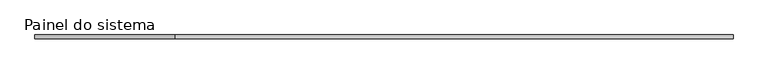
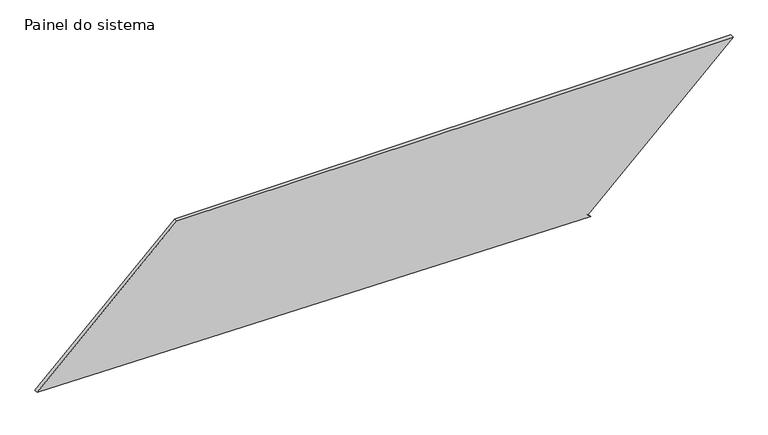
"""IFC4 building model written with IfcOpenShell, lengths in millimetres: plate geometry, Painel do sistema : Envidraçado."""

from ifc_helpers import new_model, si_unit, frame, origin, place, context, project, spatial, polyline, outline, extrude, source, transform, mapped, element, save


def painel_do_sistema_2f92d7f1(model_context):
    return source(origin(), model_context, "Body", "SweptSolid", [
        extrude(outline(polyline([(0.0, 1368.5356196), (18.146416, 1351.3394693), (933.8359883, 2317.6303845), (933.8359883, -1386.1476393), (51.1318015, -2317.6303845), (0.0, 1368.5356196)])), frame((0.0, 24.5, 0.0), z_axis=(0.0, 1.0, 0.0), x_axis=(0.0, 0.0, 1.0)), (0.0, 0.0, 1.0), 25.0),
    ])


if __name__ == "__main__":
    model = new_model("IFC4")
    model_context = context("Model", 3, world=origin())
    ifc_project = project(units=[si_unit("LENGTHUNIT", "METRE", prefix="MILLI")], contexts=[model_context])
    site = spatial("IfcSite", under=ifc_project)
    building = spatial("IfcBuilding", under=site)
    placement = place(None, origin())
    painel_do_sistema_shape = painel_do_sistema_2f92d7f1(model_context)
    element("IfcPlate", 1, ObjectType="Painel do sistema : Envidraçado", at=placement, inside=building, context=model_context, shape_type="MappedRepresentation", body=[
        mapped(painel_do_sistema_shape, transform((0.0, 0.0, 0.0), x_axis=(1.0, 0.0, 0.0), y_axis=(0.0, 1.0, 0.0), z_axis=(0.0, 0.0, 1.0))),
    ])
    save(model, "model.ifc")

# Revit data of these elements
# Type "Painel do sistema : Envidraçado"
#   Construction Type Id = "GSP4R"
#   Analytic Construction = "Vidraça única Pilkington 1/8 pol"
#   Visual Light Transmittance = 0.9
#   Solar Heat Gain Coefficient = 0.86
#   Heat Transfer Coefficient (U) = 6.7069 W/(m²·K)
# Element 1 (IfcPlate, "Painel do sistema : Envidraçado")
#   Materials on its faces: "Vidro"
# Materials
#   "Vidro": class "Vidro", colour RGB 0 128 192, transparency 0.9, Description = "Vidro de sílica", Cost = 0
